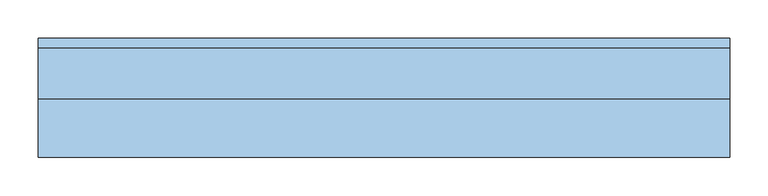
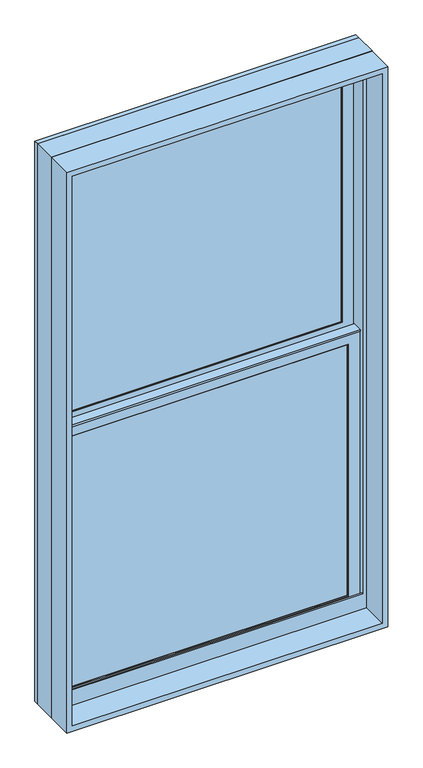
"""IFC4 building model written with IfcOpenShell, lengths in millimetres: window geometry, Window-Double_Hung-Marvin-Essential : ESDH3056."""

import ifcopenshell
import ifcopenshell.guid

model = None  # the IFC model being written
_history = None  # IfcOwnerHistory: only IFC2X3 demands one
_inside = {}  # id of a spatial element -> (the spatial element, [elements in it])
_under = {}  # id of a project, library or spatial element -> (it, [spatial elements below it])
_declared = {}  # id of a project -> (the project, [libraries it declares])
_typed = {}  # id of a type object -> (the type object, [elements of that type])
_made_of = {}  # id of a material, layer set ... -> (it, [elements and type objects made of it])


def new_model(schema):
    """Start an empty IFC model of exactly this schema.

    Asked for "IFC4X3", IfcOpenShell would pick the latest addendum, in which some entities
    have other attributes; the version numbers below select the first issue.
    IFC2X3 requires an IfcOwnerHistory on every rooted entity: one is made here for all.
    """
    global model, _history
    if schema == "IFC4X3":
        model = ifcopenshell.file(schema_version=(4, 3, 0, 0))
    else:
        model = ifcopenshell.file(schema=schema)
    _inside.clear()
    _under.clear()
    _declared.clear()
    _typed.clear()
    _made_of.clear()
    _history = None
    if model.schema == "IFC2X3":
        org = make("IfcOrganization", Name="unknown")
        user = make(
            "IfcPersonAndOrganization",
            ThePerson=make("IfcPerson", FamilyName="unknown"),
            TheOrganization=org,
        )
        app = make(
            "IfcApplication",
            ApplicationDeveloper=org,
            Version="unknown",
            ApplicationFullName="unknown",
            ApplicationIdentifier="unknown",
        )
        _history = make(
            "IfcOwnerHistory",
            OwningUser=user,
            OwningApplication=app,
            ChangeAction="ADDED",
            CreationDate=0,
        )
    return model


def make(cls, **values):
    """One entity of the class cls with the attributes given. An attribute that is None is left unset."""
    return model.create_entity(
        cls, **{name: value for name, value in values.items() if value is not None}
    )


def rooted(cls, **values):
    """An entity with a GlobalId (a new one), such as an element, a storey or a relation."""
    return make(cls, GlobalId=ifcopenshell.guid.new(), OwnerHistory=_history, **values)


def si_unit(unit_type, name, prefix=None):
    """IfcSIUnit, for example si_unit("LENGTHUNIT", "METRE", prefix="MILLI")."""
    return make("IfcSIUnit", UnitType=unit_type, Prefix=prefix, Name=name)


def assignment(units):
    """IfcUnitAssignment: the units of a project."""
    return None if units is None else make("IfcUnitAssignment", Units=units)


def point(xyz):
    """IfcCartesianPoint."""
    return None if xyz is None else make("IfcCartesianPoint", Coordinates=xyz)


def direction(xyz):
    """IfcDirection."""
    return None if xyz is None else make("IfcDirection", DirectionRatios=xyz)


def frame(location, z_axis=None, x_axis=None):
    """IfcAxis2Placement3D, a coordinate frame: its origin and axes. An axis left out is left unset."""
    return make(
        "IfcAxis2Placement3D",
        Location=point(location),
        Axis=direction(z_axis),
        RefDirection=direction(x_axis),
    )


def origin():
    """The frame at (0, 0, 0) with its axes left unset."""
    return frame((0.0, 0.0, 0.0))


def place(relative_to, where):
    """IfcLocalPlacement: puts the frame where relative to a parent placement (None: the world)."""
    return make(
        "IfcLocalPlacement", PlacementRelTo=relative_to, RelativePlacement=where
    )


def context(
    kind, dimensions, precision=None, world=None, true_north=None, identifier=None
):
    """IfcGeometricRepresentationContext, for example the 3D "Model" context."""
    return make(
        "IfcGeometricRepresentationContext",
        ContextIdentifier=identifier,
        ContextType=kind,
        CoordinateSpaceDimension=dimensions,
        Precision=precision,
        WorldCoordinateSystem=world,
        TrueNorth=true_north,
    )


def project(units=None, contexts=None):
    """IfcProject with its units and contexts."""
    return rooted(
        "IfcProject",
        Name="project",
        RepresentationContexts=contexts,
        UnitsInContext=assignment(units),
    )


def spatial(cls, under=None, at=None, **own):
    """A site, building, storey or space (cls), placed at a placement, below another one or the project."""
    s = rooted(cls, ObjectPlacement=at, **own)
    if under is not None:
        _under.setdefault(under.id(), (under, []))[1].append(s)
    return s


def polyline(points):
    """IfcPolyline through the points."""
    return make("IfcPolyline", Points=[point(p) for p in points])


def outline(outer, holes=None, kind="AREA"):
    """IfcArbitraryClosedProfileDef: a profile drawn as a closed curve; with holes, ...WithVoids."""
    if holes is None:
        return make("IfcArbitraryClosedProfileDef", ProfileType=kind, OuterCurve=outer)
    return make(
        "IfcArbitraryProfileDefWithVoids",
        ProfileType=kind,
        OuterCurve=outer,
        InnerCurves=holes,
    )


def extrude(swept, where, along, depth):
    """IfcExtrudedAreaSolid: the profile swept, set in the frame where, extruded along a direction by depth."""
    return make(
        "IfcExtrudedAreaSolid",
        SweptArea=swept,
        Position=where,
        ExtrudedDirection=direction(along),
        Depth=depth,
    )


def faces_of(points, faces, orient=None, outer=None):
    """IfcFace entities. A face is a list of loops; a loop is a list of indices into points, from 0.

    orient and outer hold one flag for each loop. By default every Orientation is true, the
    first loop of a face is its IfcFaceOuterBound and the others are IfcFaceBound.
    """
    made = []
    for i, loops in enumerate(faces):
        bounds = []
        for j, loop in enumerate(loops):
            is_outer = j == 0 if outer is None else outer[i][j]
            bounds.append(
                make(
                    "IfcFaceOuterBound" if is_outer else "IfcFaceBound",
                    Bound=make("IfcPolyLoop", Polygon=[points[k] for k in loop]),
                    Orientation=True if orient is None else orient[i][j],
                )
            )
        made.append(make("IfcFace", Bounds=bounds))
    return made


def faceted_brep(points, faces, orient=None, outer=None, voids=None):
    """IfcFacetedBrep: a solid bounded by flat faces; with voids (closed shells), ...WithVoids."""
    shared = [point(p) for p in points]
    hull = make("IfcClosedShell", CfsFaces=faces_of(shared, faces, orient, outer))
    if voids is None:
        return make("IfcFacetedBrep", Outer=hull)
    return make(
        "IfcFacetedBrepWithVoids",
        Outer=hull,
        Voids=[
            make(cls, CfsFaces=faces_of(shared, fs, o, b)) for cls, fs, o, b in voids
        ],
    )


def shape(context_of_items, identifier, shape_type, items):
    """IfcShapeRepresentation: the items that make up one representation, for example the "Body"."""
    return make(
        "IfcShapeRepresentation",
        ContextOfItems=context_of_items,
        RepresentationIdentifier=identifier,
        RepresentationType=shape_type,
        Items=items,
    )


def source(mapping_origin, context_of_items, identifier, shape_type, items):
    """IfcRepresentationMap: a shape defined once, which mapped items show again and again."""
    return make(
        "IfcRepresentationMap",
        MappingOrigin=mapping_origin,
        MappedRepresentation=shape(context_of_items, identifier, shape_type, items),
    )


def transform(
    local_origin,
    x_axis=None,
    y_axis=None,
    z_axis=None,
    scale=None,
    scale2=None,
    scale3=None,
    uniform=True,
):
    """IfcCartesianTransformationOperator3D, or its non-uniform kind. x_axis, y_axis, z_axis: its Axis1, 2, 3."""
    if uniform:
        return make(
            "IfcCartesianTransformationOperator3D",
            Axis1=direction(x_axis),
            Axis2=direction(y_axis),
            LocalOrigin=point(local_origin),
            Scale=scale,
            Axis3=direction(z_axis),
        )
    return make(
        "IfcCartesianTransformationOperator3DnonUniform",
        Axis1=direction(x_axis),
        Axis2=direction(y_axis),
        LocalOrigin=point(local_origin),
        Scale=scale,
        Axis3=direction(z_axis),
        Scale2=scale2,
        Scale3=scale3,
    )


def mapped(mapping_source, mapping_target):
    """IfcMappedItem: shows the shape of a source again, moved by a transform."""
    return make(
        "IfcMappedItem", MappingSource=mapping_source, MappingTarget=mapping_target
    )


def made_of(thing, what):
    """Note that an element or type object is made of a material, layer set ...; save() writes the relation."""
    if what is not None:
        _made_of.setdefault(what.id(), (what, []))[1].append(thing)
    return thing


def element(
    cls,
    number,
    at=None,
    inside=None,
    cuts=None,
    type_object=None,
    material=None,
    context=None,
    identifier="Body",
    shape_type=None,
    held_by="IfcProductDefinitionShape",
    body=None,
    shapes=None,
    **own,
):
    """One element of the class cls, such as IfcWall. Its Tag is "e" and its number.

    at: its placement. inside: the storey or other place that contains it. cuts: it is an
    opening in that element (IfcRelVoidsElement). A single representation is given by context,
    identifier, shape_type and body (its items); several are given by shapes. held_by: the class
    of the entity that holds the representations. save() writes the other relations.
    """
    e = rooted(cls, Tag="e%d" % number, ObjectPlacement=at, **own)
    if body is not None:
        shapes = [shape(context, identifier, shape_type, body)]
    if shapes is not None:
        e.Representation = make(held_by, Representations=shapes)
    if inside is not None:
        _inside.setdefault(inside.id(), (inside, []))[1].append(e)
    if cuts is not None:
        rooted(
            "IfcRelVoidsElement", RelatingBuildingElement=cuts, RelatedOpeningElement=e
        )
    if type_object is not None:
        _typed.setdefault(type_object.id(), (type_object, []))[1].append(e)
    return made_of(e, material)


def aggregate(whole, parts):
    """IfcRelAggregates: a whole, such as a stair, and the parts it consists of."""
    return rooted("IfcRelAggregates", RelatingObject=whole, RelatedObjects=parts)


def save(model, path):
    """Write the relations noted so far, then the file.

    IfcRelAggregates (storeys below a building ...), IfcRelContainedInSpatialStructure (elements
    in a storey), IfcRelDefinesByType, IfcRelAssociatesMaterial and IfcRelDeclares: one each for
    every whole, place, type object, material and project.
    """
    for whole, parts in _under.values():
        aggregate(whole, parts)
    for where, things in _inside.values():
        rooted(
            "IfcRelContainedInSpatialStructure",
            RelatedElements=things,
            RelatingStructure=where,
        )
    for kind, things in _typed.values():
        rooted("IfcRelDefinesByType", RelatedObjects=things, RelatingType=kind)
    for what, things in _made_of.values():
        rooted("IfcRelAssociatesMaterial", RelatedObjects=things, RelatingMaterial=what)
    for by, libraries in _declared.values():
        rooted("IfcRelDeclares", RelatingContext=by, RelatedDefinitions=libraries)
    model.write(path)


def window_cffef027(model_context):
    return source(origin(), model_context, "Body", "SolidModel", [
        extrude(outline(polyline([(140.7583333, 20.6375), (140.7583333, 15.875), (121.7083333, 15.875), (121.7083333, 20.6375), (140.7583333, 20.6375)])), frame((0.0, 0.0, 831.85), z_axis=(0.0, 0.0, 1.0), x_axis=(1.0, 0.0, 0.0)), (0.0, 0.0, 1.0), 755.65),
        extrude(outline(polyline([(-121.7083333, 20.6375), (-121.7083333, 15.875), (-140.7583333, 15.875), (-140.7583333, 20.6375), (-121.7083333, 20.6375)])), frame((0.0, 0.0, 831.85), z_axis=(0.0, 0.0, 1.0), x_axis=(1.0, 0.0, 0.0)), (0.0, 0.0, 1.0), 755.65),
        extrude(outline(polyline([(393.7, 20.6375), (393.7, 15.875), (-393.7, 15.875), (-393.7, 20.6375), (393.7, 20.6375)])), frame((0.0, 0.0, 1200.15), z_axis=(0.0, 0.0, 1.0), x_axis=(1.0, 0.0, 0.0)), (0.0, 0.0, 1.0), 19.05),
        extrude(outline(polyline([(-140.7583333, 46.83125), (-140.7583333, 51.59375), (-121.7083333, 51.59375), (-121.7083333, 46.83125), (-140.7583333, 46.83125)])), frame((0.0, 0.0, 1625.6), z_axis=(0.0, 0.0, 1.0), x_axis=(1.0, 0.0, 0.0)), (0.0, 0.0, 1.0), 755.65),
        extrude(outline(polyline([(121.7083333, 46.83125), (121.7083333, 51.59375), (140.7583333, 51.59375), (140.7583333, 46.83125), (121.7083333, 46.83125)])), frame((0.0, 0.0, 1625.6), z_axis=(0.0, 0.0, 1.0), x_axis=(1.0, 0.0, 0.0)), (0.0, 0.0, 1.0), 755.65),
        extrude(outline(polyline([(-393.7, 46.83125), (-393.7, 51.59375), (393.7, 51.59375), (393.7, 46.83125), (-393.7, 46.83125)])), frame((0.0, 0.0, 1993.9), z_axis=(0.0, 0.0, 1.0), x_axis=(1.0, 0.0, 0.0)), (0.0, 0.0, 1.0), 19.05),
        extrude(outline(polyline([(140.7583333, 20.6375), (121.7083333, 20.6375), (121.7083333, 25.4), (140.7583333, 25.4), (140.7583333, 20.6375)])), frame((0.0, 0.0, 831.85), z_axis=(0.0, 0.0, 1.0), x_axis=(1.0, 0.0, 0.0)), (0.0, 0.0, 1.0), 755.65),
        extrude(outline(polyline([(-121.7083333, 20.6375), (-140.7583333, 20.6375), (-140.7583333, 25.4), (-121.7083333, 25.4), (-121.7083333, 20.6375)])), frame((0.0, 0.0, 831.85), z_axis=(0.0, 0.0, 1.0), x_axis=(1.0, 0.0, 0.0)), (0.0, 0.0, 1.0), 755.65),
        extrude(outline(polyline([(393.7, 20.6375), (-393.7, 20.6375), (-393.7, 25.4), (393.7, 25.4), (393.7, 20.6375)])), frame((0.0, 0.0, 1200.15), z_axis=(0.0, 0.0, 1.0), x_axis=(1.0, 0.0, 0.0)), (0.0, 0.0, 1.0), 19.05),
        extrude(outline(polyline([(-140.7583333, 56.35625), (-121.7083333, 56.35625), (-121.7083333, 51.59375), (-140.7583333, 51.59375), (-140.7583333, 56.35625)])), frame((0.0, 0.0, 1625.6), z_axis=(0.0, 0.0, 1.0), x_axis=(1.0, 0.0, 0.0)), (0.0, 0.0, 1.0), 755.65),
        extrude(outline(polyline([(121.7083333, 56.35625), (140.7583333, 56.35625), (140.7583333, 51.59375), (121.7083333, 51.59375), (121.7083333, 56.35625)])), frame((0.0, 0.0, 1625.6), z_axis=(0.0, 0.0, 1.0), x_axis=(1.0, 0.0, 0.0)), (0.0, 0.0, 1.0), 755.65),
        extrude(outline(polyline([(-393.7, 56.35625), (393.7, 56.35625), (393.7, 51.59375), (-393.7, 51.59375), (-393.7, 56.35625)])), frame((0.0, 0.0, 1993.9), z_axis=(0.0, 0.0, 1.0), x_axis=(1.0, 0.0, 0.0)), (0.0, 0.0, 1.0), 19.05),
        faceted_brep([(-420.6875, 5.6780605, 1617.5351748), (-420.6875, 5.6780605, 1612.9), (420.6875, 5.6780605, 1612.9), (420.6875, 5.6780605, 1617.5351748), (-420.6875, 34.8118605, 1617.5351748), (420.6875, 34.8118605, 1617.5351748), (420.6875, 34.8118605, 1612.9), (-420.6875, 34.8118605, 1612.9), (-420.6875, 30.1625, 1612.9), (-420.6875, 30.1625, 804.8625), (-420.6875, 8.9241104, 804.8625), (-420.6875, 8.9241104, 1612.9), (420.6875, 8.9241104, 1612.9), (420.6875, 30.1625, 1612.9), (420.6875, 8.9241104, 804.8625), (420.6875, 30.1625, 804.8625), (-404.8034752, 11.90625, 1598.6034752), (-404.8034752, 30.1625, 1598.6034752), (404.8034752, 30.1625, 1598.6034752), (404.8034752, 11.90625, 1598.6034752), (-388.14375, 10.4662439, 1581.94375), (-388.14375, 11.90625, 1581.94375), (388.14375, 11.90625, 1581.94375), (388.14375, 10.4662439, 1581.94375), (389.6858834, 8.9241104, 1583.4858834), (-389.6858834, 8.9241104, 1583.4858834), (404.8034752, 30.1625, 820.7465248), (404.8034752, 11.90625, 820.7465248), (388.14375, 11.90625, 837.40625), (388.14375, 10.4662439, 837.40625), (389.6858834, 8.9241104, 835.8641166), (-404.8034752, 30.1625, 820.7465248), (-404.8034752, 11.90625, 820.7465248), (-388.14375, 11.90625, 837.40625), (-388.14375, 10.4662439, 837.40625), (-389.6858834, 8.9241104, 835.8641166)], [[[0, 1, 2, 3]], [[4, 5, 6, 7]], [[1, 0, 4, 7, 8, 9, 10, 11]], [[2, 1, 11, 12]], [[7, 6, 13, 8]], [[3, 2, 12, 14, 15, 13, 6, 5]], [[0, 3, 5, 4]], [[16, 17, 18, 19]], [[20, 21, 22, 23]], [[20, 23, 24, 25]], [[19, 18, 26, 27]], [[23, 22, 28, 29]], [[24, 23, 29, 30]], [[27, 26, 31, 32]], [[29, 28, 33, 34]], [[30, 29, 34, 35]], [[15, 14, 10, 9]], [[15, 9, 8, 13], [18, 17, 31, 26]], [[17, 16, 32, 31]], [[16, 19, 27, 32], [22, 21, 33, 28]], [[21, 20, 34, 33]], [[20, 25, 35, 34]], [[10, 14, 12, 11], [25, 24, 30, 35]]]),
        extrude(outline(polyline([(38.5955581, 1598.6125), (33.5778968, 1598.6125), (33.5778968, 1600.2), (39.9405976, 1600.2), (39.9405976, 1598.6125), (61.515625, 1598.6125), (47.6307501, 1595.2975159), (38.5955581, 1595.2975159), (38.5955581, 1598.6125)])), frame((-420.6875, 0.0, 0.0), z_axis=(1.0, 0.0, 0.0), x_axis=(0.0, 1.0, 0.0)), (0.0, 0.0, 1.0), 841.375),
        faceted_brep([(450.85, 0.0, 774.7), (450.85, 0.0, 2438.4), (-450.85, 0.0, 2438.4), (-450.85, 0.0, 774.7), (424.65625, 0.0, 835.81875), (-424.65625, 0.0, 835.81875), (-424.65625, 0.0, 2412.20625), (424.65625, 0.0, 2412.20625), (424.65625, 3.96875, 774.7), (-424.65625, 3.96875, 774.7), (-424.65625, 3.96875, 835.81875), (424.65625, 3.96875, 835.81875), (-450.85, 65.6828125, 774.7), (-424.65625, 65.6828125, 774.7), (424.65625, 65.6828125, 774.7), (450.85, 65.6828125, 774.7), (-450.85, 65.6828125, 2438.4), (450.85, 65.6828125, 2438.4), (424.65625, 65.6828125, 2412.20625), (-424.65625, 65.6828125, 2412.20625)], [[[0, 1, 2, 3], [4, 5, 6, 7]], [[8, 9, 10, 11]], [[5, 4, 11, 10]], [[0, 3, 12, 13, 9, 8, 14, 15]], [[13, 12, 16, 17, 15, 14, 18, 19]], [[13, 19, 6, 5, 10, 9]], [[7, 6, 19, 18]], [[18, 14, 8, 11, 4, 7]], [[1, 0, 15, 17]], [[2, 1, 17, 16]], [[3, 2, 16, 12]]]),
        faceted_brep([(424.65625, 30.1625, 1606.55), (423.06875, 30.1625, 1606.55), (423.06875, 30.1625, 799.0544613), (424.65625, 30.1625, 799.0544613), (-423.06875, 30.1625, 1606.55), (-424.65625, 30.1625, 1606.55), (-424.65625, 30.1625, 799.0544613), (-423.06875, 30.1625, 799.0544613), (423.06875, 63.5, 1606.55), (424.65625, 63.5, 1606.55), (424.65625, 63.5, 792.5743077), (423.06875, 63.5, 792.5743077), (-424.65625, 63.5, 1606.55), (-423.06875, 63.5, 1606.55), (-423.06875, 63.5, 792.5743077), (-424.65625, 63.5, 792.5743077), (435.9108932, 3.96875, 804.1460105), (435.9108932, 3.96875, 774.7), (435.9108932, 65.6828125, 774.7), (435.9108932, 65.6828125, 792.150012), (-435.9108932, 3.96875, 774.7), (-435.9108932, 3.96875, 804.1460105), (-435.9108932, 65.6828125, 792.150012), (-435.9108932, 65.6828125, 774.7), (435.9108932, 78.58125, 789.6428097), (-435.9108932, 78.58125, 789.6428097), (-433.8971252, 68.2348864, 791.6539391), (-415.93135, 68.2348864, 791.6539391), (-415.93135, 65.6828125, 792.150012), (415.93135, 65.6828125, 792.150012), (415.93135, 68.2348864, 791.6539391), (433.8971252, 68.2348864, 791.6539391), (-450.85, 65.6828125, 774.7), (-450.85, 78.5948249, 774.7), (450.85, 78.5948249, 774.7), (450.85, 65.6828125, 774.7), (-450.85, 78.58125, 2438.4), (450.85, 78.58125, 2438.4), (435.9108932, 78.58125, 2423.4608932), (-435.9108932, 78.58125, 2423.4608932), (-450.85, 65.6828125, 2438.4), (-433.8971252, 68.2348864, 2421.4471252), (433.8971252, 68.2348864, 2421.4471252), (415.93135, 68.2348864, 2403.48135), (-415.93135, 68.2348864, 2403.48135), (-415.93135, 65.6828125, 2403.48135), (415.93135, 65.6828125, 2403.48135), (450.85, 65.6828125, 2438.4)], [[[0, 1, 2, 3]], [[4, 5, 6, 7]], [[8, 9, 10, 11]], [[12, 13, 14, 15]], [[1, 8, 11, 2]], [[9, 0, 3, 10]], [[1, 0, 9, 8]], [[5, 4, 13, 12]], [[5, 12, 15, 6]], [[13, 4, 7, 14]], [[16, 17, 18, 19]], [[20, 21, 22, 23]], [[24, 25, 26, 27, 28, 22, 21, 16, 19, 29, 30, 31], [3, 2, 11, 10], [7, 6, 15, 14]], [[17, 16, 21, 20]], [[17, 20, 23, 32, 33, 34, 35, 18]], [[34, 33, 36, 37], [25, 24, 38, 39]], [[33, 32, 40, 36]], [[39, 41, 26, 25]], [[41, 42, 31, 30, 43, 44, 27, 26]], [[44, 45, 28, 27]], [[40, 32, 23, 22, 28, 45, 46, 29, 19, 18, 35, 47]], [[36, 40, 47, 37]], [[39, 38, 42, 41]], [[44, 43, 46, 45]], [[34, 37, 47, 35]], [[42, 38, 24, 31]], [[46, 43, 30, 29]]]),
        extrude(outline(polyline([(400.84375, 11.90625), (-400.84375, 11.90625), (-400.84375, 15.08125), (400.84375, 15.08125), (400.84375, 11.90625)])), frame((0.0, 0.0, 824.70625), z_axis=(0.0, 0.0, 1.0), x_axis=(1.0, 0.0, 0.0)), (0.0, 0.0, 1.0), 769.9375),
        extrude(outline(polyline([(400.84375, 42.8625), (-400.84375, 42.8625), (-400.84375, 46.0375), (400.84375, 46.0375), (400.84375, 42.8625)])), frame((0.0, 0.0, 1618.45625), z_axis=(0.0, 0.0, 1.0), x_axis=(1.0, 0.0, 0.0)), (0.0, 0.0, 1.0), 769.9375),
        faceted_brep([(-388.14375, 31.194477, 1581.94375), (-389.6858834, 32.7366104, 1583.4858834), (389.6858834, 32.7366104, 1583.4858834), (388.14375, 31.194477, 1581.94375), (-388.14375, 30.1625, 1581.94375), (388.14375, 30.1625, 1581.94375), (-420.6875, 32.7366104, 1614.4875), (-420.6875, 30.1625, 1614.4875), (420.6875, 30.1625, 1614.4875), (420.6875, 32.7366104, 1614.4875), (389.6858834, 32.7366104, 835.8641166), (388.14375, 31.194477, 837.40625), (388.14375, 30.1625, 837.40625), (420.6875, 30.1625, 804.8625), (420.6875, 32.7366104, 804.8625), (-389.6858834, 32.7366104, 835.8641166), (-388.14375, 31.194477, 837.40625), (-388.14375, 30.1625, 837.40625), (-420.6875, 30.1625, 804.8625), (-420.6875, 32.7366104, 804.8625)], [[[0, 1, 2, 3]], [[4, 0, 3, 5]], [[6, 7, 8, 9]], [[3, 2, 10, 11]], [[5, 3, 11, 12]], [[9, 8, 13, 14]], [[11, 10, 15, 16]], [[12, 11, 16, 17]], [[14, 13, 18, 19]], [[9, 14, 19, 6], [1, 15, 10, 2]], [[16, 15, 1, 0]], [[17, 16, 0, 4]], [[7, 18, 13, 8], [5, 12, 17, 4]], [[19, 18, 7, 6]]]),
        faceted_brep([(-404.8034752, 42.8625, 2392.3534752), (-404.8034752, 61.11875, 2392.3534752), (404.8034752, 61.11875, 2392.3534752), (404.8034752, 42.8625, 2392.3534752), (-388.14375, 41.4224939, 2375.69375), (-388.14375, 42.8625, 2375.69375), (388.14375, 42.8625, 2375.69375), (388.14375, 41.4224939, 2375.69375), (-389.6858834, 39.8803604, 2377.2358834), (389.6858834, 39.8803604, 2377.2358834), (-420.6875, 61.11875, 2408.2375), (-420.6875, 39.8803604, 2408.2375), (420.6875, 39.8803604, 2408.2375), (420.6875, 61.11875, 2408.2375), (404.8034752, 61.11875, 1614.4965248), (404.8034752, 42.8625, 1614.4965248), (388.14375, 42.8625, 1631.15625), (388.14375, 41.4224939, 1631.15625), (389.6858834, 39.8803604, 1629.6141166), (420.6875, 39.8803604, 1598.6125), (420.6875, 61.11875, 1598.6125), (-404.8034752, 61.11875, 1614.4965248), (-404.8034752, 42.8625, 1614.4965248), (-388.14375, 42.8625, 1631.15625), (-388.14375, 41.4224939, 1631.15625), (-389.6858834, 39.8803604, 1629.6141166), (-420.6875, 39.8803604, 1598.6125), (-420.6875, 61.11875, 1598.6125)], [[[0, 1, 2, 3]], [[4, 5, 6, 7]], [[8, 4, 7, 9]], [[10, 11, 12, 13]], [[3, 2, 14, 15]], [[7, 6, 16, 17]], [[9, 7, 17, 18]], [[13, 12, 19, 20]], [[15, 14, 21, 22]], [[17, 16, 23, 24]], [[18, 17, 24, 25]], [[20, 19, 26, 27]], [[13, 20, 27, 10], [1, 21, 14, 2]], [[22, 21, 1, 0]], [[3, 15, 22, 0], [5, 23, 16, 6]], [[24, 23, 5, 4]], [[25, 24, 4, 8]], [[11, 26, 19, 12], [9, 18, 25, 8]], [[27, 26, 11, 10]]]),
        faceted_brep([(-420.6875, 61.11875, 1598.6125), (-420.6875, 63.6928604, 1598.6125), (420.6875, 63.6928604, 1598.6125), (420.6875, 61.11875, 1598.6125), (-388.14375, 62.150727, 1631.15625), (-388.14375, 61.11875, 1631.15625), (388.14375, 61.11875, 1631.15625), (388.14375, 62.150727, 1631.15625), (-389.6858834, 63.6928604, 1629.6141166), (389.6858834, 63.6928604, 1629.6141166), (420.6875, 63.6928604, 2408.2375), (420.6875, 61.11875, 2408.2375), (388.14375, 61.11875, 2375.69375), (388.14375, 62.150727, 2375.69375), (389.6858834, 63.6928604, 2377.2358834), (-420.6875, 63.6928604, 2408.2375), (-420.6875, 61.11875, 2408.2375), (-388.14375, 61.11875, 2375.69375), (-388.14375, 62.150727, 2375.69375), (-389.6858834, 63.6928604, 2377.2358834)], [[[0, 1, 2, 3]], [[4, 5, 6, 7]], [[8, 4, 7, 9]], [[3, 2, 10, 11]], [[7, 6, 12, 13]], [[9, 7, 13, 14]], [[11, 10, 15, 16]], [[13, 12, 17, 18]], [[14, 13, 18, 19]], [[16, 15, 1, 0]], [[3, 11, 16, 0], [5, 17, 12, 6]], [[18, 17, 5, 4]], [[19, 18, 4, 8]], [[1, 15, 10, 2], [9, 14, 19, 8]]]),
        extrude(outline(polyline([(400.84375, 26.19375), (-400.84375, 26.19375), (-400.84375, 30.1625), (400.84375, 30.1625), (400.84375, 26.19375)])), frame((0.0, 0.0, 824.70625), z_axis=(0.0, 0.0, 1.0), x_axis=(1.0, 0.0, 0.0)), (0.0, 0.0, 1.0), 769.9375),
        extrude(outline(polyline([(400.84375, 57.15), (-400.84375, 57.15), (-400.84375, 61.11875), (400.84375, 61.11875), (400.84375, 57.15)])), frame((0.0, 0.0, 1618.45625), z_axis=(0.0, 0.0, 1.0), x_axis=(1.0, 0.0, 0.0)), (0.0, 0.0, 1.0), 769.9375),
        extrude(outline(polyline([(2438.4, 450.85), (2438.4, -450.85), (774.7, -450.85), (774.7, 450.85), (2438.4, 450.85)]), holes=[polyline([(2422.525, 434.975), (790.575, 434.975), (790.575, -434.975), (2422.525, -434.975), (2422.525, 434.975)])]), frame((0.0, -76.2, 0.0), z_axis=(0.0, 1.0, 0.0), x_axis=(0.0, 0.0, 1.0)), (0.0, 0.0, 1.0), 75.40625),
    ])


if __name__ == "__main__":
    model = new_model("IFC4")
    model_context = context("Model", 3, world=origin())
    ifc_project = project(units=[si_unit("LENGTHUNIT", "METRE", prefix="MILLI")], contexts=[model_context])
    site = spatial("IfcSite", under=ifc_project)
    building = spatial("IfcBuilding", under=site)
    placement = place(None, origin())
    window_shape = window_cffef027(model_context)
    element("IfcWindow", 1, ObjectType="Window-Double_Hung-Marvin-Essential : ESDH3056", at=placement, inside=building, context=model_context, shape_type="MappedRepresentation", body=[
        mapped(window_shape, transform((0.0, 0.0, 0.0), x_axis=(1.0, 0.0, 0.0), y_axis=(0.0, 1.0, 0.0), z_axis=(0.0, 0.0, 1.0))),
    ])
    save(model, "model.ifc")

# Revit data of these elements
# Type "Window-Double_Hung-Marvin-Essential : ESDH3056"
#   Type Mark = "72"
#   Window Type = "Essential Double Hung"
#   Product data url = "https://bimobject.com/marvin-windows-and-doors/product/marvin-dhwau"
#   Product Guid = "c4a96547-874c-4385-91dc-a058adc19d98"
#   Frame = "All Ultrex"
#   Egress Window = "Yes"
#   URL = "www.marvin.com"
#   Model = "ESDH3056"
#   Manufacturer = "Marvin Windows and Doors"
#   Label Egress = "EGRESS WDW"
#   Glass Type = "IG Low E II with Argon"
#   Design Pressure = "DP40"
#   Description = "3666 DBHG"
#   Analytic Construction = "<None>"
#   Prairie Corner Width = 0' - 4"
#   Prairie Corner Height = 0' - 4"
#   Egress Width = 2' - 8 9/16"
#   Egress Height = 2' - 4 27/128"
#   Rough Width = 3' - 0"
#   Rough Height = 5' - 6"
#   Nominal Width = 3' - 0"
#   Nominal Height = 5' - 6"
#   Inset to Installation Flange [instance default] = 0' - 1"
#   Height = 5' - 5 1/2"
#   Egress Area = 6.3793 SF
#   Default Head Height = 8' - 0"
#   Width = 2' - 11 1/2"
#   Daylight Area = 12.4425 SF
#   DLO Width = 2' - 6 9/16"
#   DLO Height = 2' - 5 5/16"
#   Muntins Top Sash = yes
#   Lites Wide Top Sash = 3
#   Lites Wide Bottom Sash = 3
#   Lites High Top Sash = 2
#   Lites High Bottom Sash = 2
#   Lite Cut Prairie 9 = no
#   Lite Cut HV Grid = yes
#   Muntins Bottom Sash = yes
#   Label Visibility = no
#   Jamb Extension Visibility = yes
#   Edition number = 1
#   Interior Material = Ultrex-Marvin-Stonewhite
#   Glazing Material = Glass-Marvin-IG Low E II with Argon
#   Cladding Material = Ultrex-Marvin-Pebblegray
#   Wall Closure = (empty or 0)
#   Assembly Code = ""
# Element 1 (IfcWindow, "Window-Double_Hung-Marvin-Essential : ESDH3056")
#   Materials on its faces: "Ultrex-Marvin-Pebblegray", "Ultrex-Marvin-Stonewhite", "Glass-Marvin-IG Low E II with Argon"
# Materials
#   "Ultrex-Marvin-Stonewhite": class "Paint", colour RGB 250 251 245, transparency 0
#   "Glass-Marvin-IG Low E II with Argon": class "Glass", colour RGB 0 128 192, transparency 0.85
#   "Ultrex-Marvin-Pebblegray": class "Paint", colour RGB 189 185 173, transparency 0
